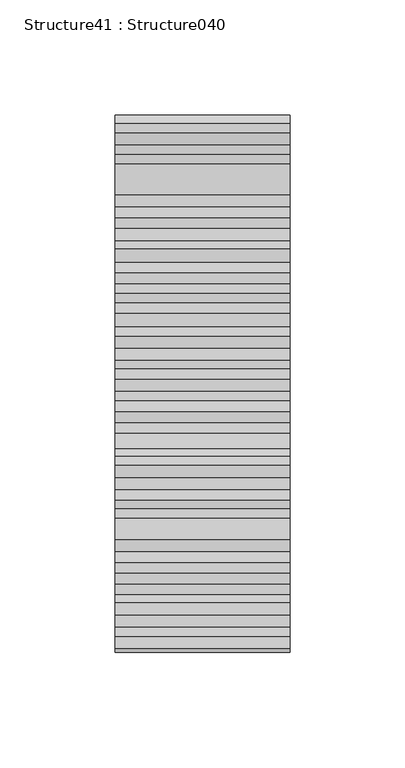
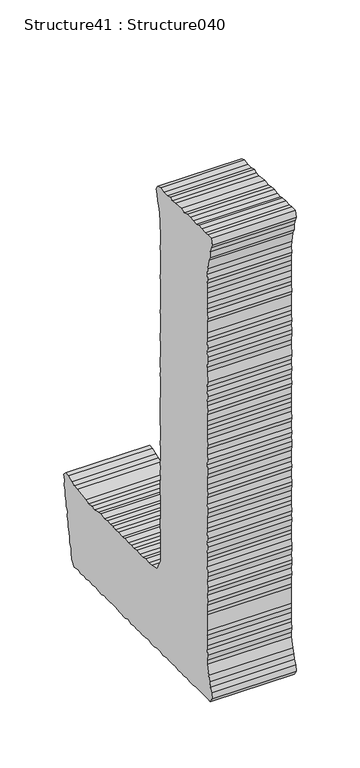
"""IFC4 building model written with IfcOpenShell, lengths in millimetres: proxy geometry, Structure41 : Structure040."""

from ifc_helpers import new_model, si_unit, frame, origin, place, context, project, spatial, polyline, outline, extrude, source, transform, mapped, element, save


def structure41_structure040_c025b67e(model_context):
    return source(origin(), model_context, "Body", "SweptSolid", [
        extrude(outline(polyline([(255834.0417556, 3629.5984101), (255832.2815044, 3625.472972), (255832.8832311, 3619.6145609), (255831.1213754, 3616.0972679), (255831.1213754, 3611.4134274), (255829.9403865, 3605.572667), (255829.9403865, 3601.4536473), (255827.5784087, 3597.9540049), (255828.1801353, 3593.2541183), (255826.4423487, 3587.9685511), (255826.4423487, 3583.8864372), (255825.2613598, 3578.6104977), (255824.0787663, 3574.5107332), (255824.0787663, 3569.8268927), (255822.3185151, 3565.7094775), (255821.7392529, 3561.025637), (255821.1375262, 3555.7416744), (255817.0586216, 3550.4833855), (255811.198606, 3551.6675836), (255807.0747724, 3550.4833855), (255801.8148789, 3551.0658569), (255798.2943766, 3550.4833855), (255793.6137453, 3551.6675836), (255788.9347186, 3551.0658569), (255783.6523606, 3551.6675836), (255778.9717293, 3550.4833855), (255773.6909759, 3550.4833855), (255770.168869, 3551.6675836), (255765.4898423, 3551.0658569), (255760.7867465, 3551.0658569), (255756.7078419, 3551.6675836), (255752.0063507, 3551.6675836), (255746.1447305, 3550.4833855), (255736.7850725, 3550.4833855), (255732.6837034, 3551.6675836), (255727.4013454, 3550.4833855), (255722.6998542, 3551.0658569), (255719.2002118, 3550.4833855), (255713.9419229, 3551.0658569), (255710.3973515, 3550.4833855), (255705.137458, 3551.0658569), (255700.4359668, 3551.6675836), (255695.7553355, 3550.4833855), (255691.6780355, 3550.4833855), (255686.9749397, 3551.6675836), (255682.2943084, 3551.6675836), (255676.9910906, 3550.4833855), (255671.731197, 3551.6675836), (255668.2315546, 3551.0658569), (255662.9508012, 3551.6675836), (255657.6684432, 3551.6675836), (255654.1704054, 3550.4833855), (255649.4673096, 3551.0658569), (255644.2074161, 3551.0658569), (255640.1076516, 3551.6675836), (255636.0062825, 3550.4833855), (255631.3047914, 3550.4833855), (255625.4431711, 3551.6675836), (255606.699786, 3551.6675836), (255603.1792838, 3551.0658569), (255600.2589036, 3555.7416744), (255601.4190326, 3561.025637), (255603.1792838, 3565.1254015), (255604.3602727, 3569.8268927), (255605.5187971, 3575.0851816), (255608.4600371, 3583.8864372), (255608.4600371, 3587.9685511), (255607.3015127, 3593.2541183), (255607.8583105, 3598.5284533), (255607.8583105, 3602.0280957), (255608.4600371, 3607.3393366), (255607.8583105, 3612.0135494), (255608.4600371, 3616.0972679), (255608.4600371, 3631.3410106), (255607.8583105, 3634.856699), (255608.4600371, 3640.7167147), (255607.3015127, 3644.8245022), (255608.4600371, 3650.1004418), (255607.3015127, 3654.7842823), (255607.3015127, 3658.3015753), (255608.4600371, 3662.9854159), (255607.3015127, 3668.8261762), (255607.3015127, 3672.3691429), (255607.8583105, 3678.2018803), (255608.4600371, 3682.8857208), (255608.4600371, 3686.4030139), (255607.8583105, 3691.0868544), (255607.3015127, 3696.9709391), (255607.8583105, 3701.0723082), (255607.3015127, 3705.1720727), (255607.8583105, 3711.0304837), (255607.8583105, 3715.1302482), (255608.4600371, 3719.2316172), (255608.4600371, 3724.4979292), (255607.3015127, 3729.7738688), (255607.3015127, 3733.2991849), (255607.8583105, 3737.9750024), (255608.4600371, 3743.8414364), (255607.3015127, 3747.9428055), (255608.4600371, 3752.04257), (255607.8583105, 3756.7440611), (255608.4600371, 3762.5848215), (255607.3015127, 3767.2590344), (255607.3015127, 3771.9605256), (255607.8583105, 3776.0618947), (255607.3015127, 3780.7441306), (255608.4600371, 3784.8438951), (255608.4600371, 3790.7039107), (255607.3015127, 3794.8309535), (255608.4600371, 3800.0876378), (255607.8583105, 3804.7730829), (255607.8583105, 3809.4729695), (255608.4600371, 3812.9726119), (255607.8583105, 3817.6741031), (255608.4600371, 3823.5341187), (255607.3015127, 3827.6162325), (255608.4600371, 3832.3161191), (255607.8583105, 3836.4174882), (255607.3015127, 3841.6741725), (255607.8583105, 3846.3772683), (255607.8583105, 3850.4754282), (255607.3015127, 3855.1769193), (255608.4600371, 3864.5446004), (255607.8583105, 3869.2444869), (255607.3015127, 3875.0772243), (255607.3015127, 3879.1769888), (255607.8583105, 3883.8881076), (255607.3015127, 3887.9621984), (255607.8583105, 3893.822214), (255607.8583105, 3897.3475301), (255608.4600371, 3902.0201384), (255608.4600371, 3912.5896682), (255607.3015127, 3916.0909152), (255608.4600371, 3921.3748778), (255607.8583105, 3925.4746423), (255607.8583105, 3930.1745289), (255608.4600371, 3935.4328178), (255608.4600371, 3940.718385), (255607.8583105, 3945.4182716), (255607.8583105, 3950.0940891), (255607.3015127, 3953.5937315), (255607.8583105, 3958.8776941), (255607.3015127, 3964.1343784), (255606.1205238, 3972.9372387), (255603.758546, 3977.0209571), (255603.1792838, 3982.8793681), (255602.0207593, 3987.5792547), (255600.2589036, 3991.0788971), (255602.0207593, 3996.9645864), (255607.3015127, 3996.9645864), (255611.3804173, 3996.390138), (255616.6627753, 3996.9645864), (255621.9435287, 3996.9645864), (255625.4431711, 3995.7803883), (255630.1221978, 3996.390138), (255634.8252936, 3996.9645864), (255639.5059249, 3996.9645864), (255644.2074161, 3995.7803883), (255649.4673096, 3996.9645864), (255658.8494321, 3995.7803883), (255662.9508012, 3995.7803883), (255666.4713035, 3996.9645864), (255671.1519348, 3995.7803883), (255676.4342928, 3995.7803883), (255681.6925817, 3996.9645864), (255685.7939508, 3995.7803883), (255688.7351909, 3991.6806238), (255686.9749397, 3987.0048063), (255685.7939508, 3981.7208437), (255684.6129619, 3977.6194746), (255682.8735706, 3972.3627903), (255682.2943084, 3962.9774586), (255682.2943084, 3958.8776941), (255681.6925817, 3953.5937315), (255681.6925817, 3943.6339514), (255682.2943084, 3940.1166583), (255681.1133195, 3934.2758979), (255681.1133195, 3925.4746423), (255681.6925817, 3920.7908018), (255681.1133195, 3915.5068392), (255682.2943084, 3911.4054701), (255681.1133195, 3906.7328618), (255681.1133195, 3901.44569), (255681.6925817, 3896.763454), (255681.6925817, 3887.38775), (255681.1133195, 3882.7039095), (255682.2943084, 3878.0024183), (255681.1133195, 3874.5043805), (255681.1133195, 3865.1190488), (255681.6925817, 3860.4432313), (255682.2943084, 3854.5751926), (255681.1133195, 3845.1914656), (255681.1133195, 3841.0900965), (255681.6925817, 3836.4174882), (255682.2943084, 3832.3161191), (255682.2943084, 3827.0321565), (255681.1133195, 3821.7722629), (255682.2943084, 3818.2309008), (255681.6925817, 3812.9726119), (255681.6925817, 3808.290376), (255681.1133195, 3803.0064134), (255681.1133195, 3798.3305959), (255682.2943084, 3793.6451507), (255682.2943084, 3770.8036057), (255681.6925817, 3766.1021146), (255681.1133195, 3760.2437036), (255681.6925817, 3756.7440611), (255682.2943084, 3752.04257), (255681.1133195, 3746.7586074), (255681.6925817, 3742.0747668), (255681.6925817, 3736.7988273), (255682.2943084, 3732.1149867), (255681.6925817, 3728.0152223), (255682.2943084, 3723.9154578), (255681.6925817, 3718.0554422), (255682.2943084, 3713.3555556), (255682.2943084, 3704.0135482), (255681.1133195, 3700.4705815), (255681.6925817, 3695.786741), (255681.6925817, 3681.7271964), (255682.2943084, 3676.4432338), (255682.2943084, 3672.3691429), (255681.1133195, 3666.5027089), (255681.6925817, 3662.9854159), (255681.6925817, 3652.9999621), (255681.1133195, 3648.9258713), (255681.1133195, 3643.0578326), (255681.6925817, 3638.9580681), (255685.2146886, 3631.3410106), (255686.9749397, 3627.8397636), (255695.7553355, 3626.0554434), (255700.4359668, 3625.472972), (255705.137458, 3626.6571701), (255709.8180893, 3625.472972), (255713.9419229, 3625.472972), (255719.2002118, 3626.0554434), (255723.8808431, 3625.472972), (255727.4013454, 3626.0554434), (255732.6837034, 3625.472972), (255737.9435969, 3626.6571701), (255742.0433614, 3625.472972), (255747.9049816, 3626.0554434), (255752.5856129, 3625.472972), (255756.7078419, 3626.6571701), (255760.7867465, 3626.0554434), (255765.4898423, 3626.6571701), (255770.168869, 3625.472972), (255776.0304892, 3626.6571701), (255779.5509915, 3626.0554434), (255784.810885, 3625.472972), (255789.4915163, 3626.0554434), (255794.1930075, 3625.472972), (255799.4753655, 3626.0554434), (255812.9363926, 3627.8397636), (255817.0586216, 3628.998288), (255821.1375262, 3630.1824862), (255826.4423487, 3632.5155811), (255830.5196487, 3633.0980525), (255834.0417556, 3629.5984101)])), frame((-38594.2176606, 0.0, 0.0), z_axis=(1.0, 0.0, 0.0), x_axis=(0.0, 1.0, 0.0)), (0.0, 0.0, 1.0), 76.2),
    ])


if __name__ == "__main__":
    model = new_model("IFC4")
    model_context = context("Model", 3, world=origin())
    ifc_project = project(units=[si_unit("LENGTHUNIT", "METRE", prefix="MILLI")], contexts=[model_context])
    site = spatial("IfcSite", under=ifc_project)
    building = spatial("IfcBuilding", under=site)
    placement = place(None, origin())
    structure41_structure040_shape = structure41_structure040_c025b67e(model_context)
    element("IfcBuildingElementProxy", 1, Name="Structure41 : Structure040", ObjectType="Structure41 : Structure040", at=placement, inside=building, context=model_context, shape_type="MappedRepresentation", body=[
        mapped(structure41_structure040_shape, transform((0.0, 0.0, 0.0), x_axis=(1.0, 0.0, 0.0), y_axis=(0.0, 1.0, 0.0), z_axis=(0.0, 0.0, 1.0))),
    ])
    save(model, "model.ifc")

# Revit data of these elements
# Type "Structure41 : Structure040"
#   NameOverride = "Structure040"
# Element 1 (IfcBuildingElementProxy, "Structure41 : Structure040")
#   Materials on its faces: "BRUSHED ALUM. LETTERING"
# Materials
#   "BRUSHED ALUM. LETTERING": class "Unassigned", colour RGB 169 181 186, transparency 0, Cost = 0
